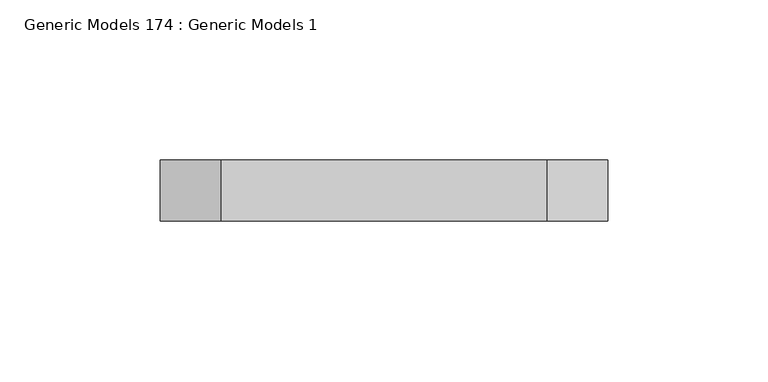
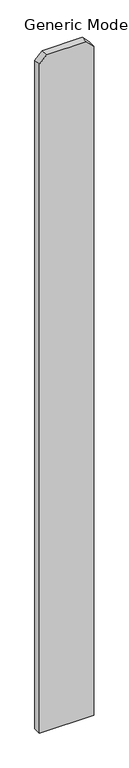
"""IFC4 building model written with IfcOpenShell, lengths in millimetres: proxy geometry, Generic Models 174 : Generic Models 1."""

import ifcopenshell
import ifcopenshell.guid

model = None  # the IFC model being written
_history = None  # IfcOwnerHistory: only IFC2X3 demands one
_inside = {}  # id of a spatial element -> (the spatial element, [elements in it])
_under = {}  # id of a project, library or spatial element -> (it, [spatial elements below it])
_declared = {}  # id of a project -> (the project, [libraries it declares])
_typed = {}  # id of a type object -> (the type object, [elements of that type])
_made_of = {}  # id of a material, layer set ... -> (it, [elements and type objects made of it])


def new_model(schema):
    """Start an empty IFC model of exactly this schema.

    Asked for "IFC4X3", IfcOpenShell would pick the latest addendum, in which some entities
    have other attributes; the version numbers below select the first issue.
    IFC2X3 requires an IfcOwnerHistory on every rooted entity: one is made here for all.
    """
    global model, _history
    if schema == "IFC4X3":
        model = ifcopenshell.file(schema_version=(4, 3, 0, 0))
    else:
        model = ifcopenshell.file(schema=schema)
    _inside.clear()
    _under.clear()
    _declared.clear()
    _typed.clear()
    _made_of.clear()
    _history = None
    if model.schema == "IFC2X3":
        org = make("IfcOrganization", Name="unknown")
        user = make(
            "IfcPersonAndOrganization",
            ThePerson=make("IfcPerson", FamilyName="unknown"),
            TheOrganization=org,
        )
        app = make(
            "IfcApplication",
            ApplicationDeveloper=org,
            Version="unknown",
            ApplicationFullName="unknown",
            ApplicationIdentifier="unknown",
        )
        _history = make(
            "IfcOwnerHistory",
            OwningUser=user,
            OwningApplication=app,
            ChangeAction="ADDED",
            CreationDate=0,
        )
    return model


def make(cls, **values):
    """One entity of the class cls with the attributes given. An attribute that is None is left unset."""
    return model.create_entity(
        cls, **{name: value for name, value in values.items() if value is not None}
    )


def rooted(cls, **values):
    """An entity with a GlobalId (a new one), such as an element, a storey or a relation."""
    return make(cls, GlobalId=ifcopenshell.guid.new(), OwnerHistory=_history, **values)


def si_unit(unit_type, name, prefix=None):
    """IfcSIUnit, for example si_unit("LENGTHUNIT", "METRE", prefix="MILLI")."""
    return make("IfcSIUnit", UnitType=unit_type, Prefix=prefix, Name=name)


def assignment(units):
    """IfcUnitAssignment: the units of a project."""
    return None if units is None else make("IfcUnitAssignment", Units=units)


def point(xyz):
    """IfcCartesianPoint."""
    return None if xyz is None else make("IfcCartesianPoint", Coordinates=xyz)


def direction(xyz):
    """IfcDirection."""
    return None if xyz is None else make("IfcDirection", DirectionRatios=xyz)


def frame(location, z_axis=None, x_axis=None):
    """IfcAxis2Placement3D, a coordinate frame: its origin and axes. An axis left out is left unset."""
    return make(
        "IfcAxis2Placement3D",
        Location=point(location),
        Axis=direction(z_axis),
        RefDirection=direction(x_axis),
    )


def origin():
    """The frame at (0, 0, 0) with its axes left unset."""
    return frame((0.0, 0.0, 0.0))


def place(relative_to, where):
    """IfcLocalPlacement: puts the frame where relative to a parent placement (None: the world)."""
    return make(
        "IfcLocalPlacement", PlacementRelTo=relative_to, RelativePlacement=where
    )


def context(
    kind, dimensions, precision=None, world=None, true_north=None, identifier=None
):
    """IfcGeometricRepresentationContext, for example the 3D "Model" context."""
    return make(
        "IfcGeometricRepresentationContext",
        ContextIdentifier=identifier,
        ContextType=kind,
        CoordinateSpaceDimension=dimensions,
        Precision=precision,
        WorldCoordinateSystem=world,
        TrueNorth=true_north,
    )


def project(units=None, contexts=None):
    """IfcProject with its units and contexts."""
    return rooted(
        "IfcProject",
        Name="project",
        RepresentationContexts=contexts,
        UnitsInContext=assignment(units),
    )


def spatial(cls, under=None, at=None, **own):
    """A site, building, storey or space (cls), placed at a placement, below another one or the project."""
    s = rooted(cls, ObjectPlacement=at, **own)
    if under is not None:
        _under.setdefault(under.id(), (under, []))[1].append(s)
    return s


def polyline(points):
    """IfcPolyline through the points."""
    return make("IfcPolyline", Points=[point(p) for p in points])


def outline(outer, holes=None, kind="AREA"):
    """IfcArbitraryClosedProfileDef: a profile drawn as a closed curve; with holes, ...WithVoids."""
    if holes is None:
        return make("IfcArbitraryClosedProfileDef", ProfileType=kind, OuterCurve=outer)
    return make(
        "IfcArbitraryProfileDefWithVoids",
        ProfileType=kind,
        OuterCurve=outer,
        InnerCurves=holes,
    )


def extrude(swept, where, along, depth):
    """IfcExtrudedAreaSolid: the profile swept, set in the frame where, extruded along a direction by depth."""
    return make(
        "IfcExtrudedAreaSolid",
        SweptArea=swept,
        Position=where,
        ExtrudedDirection=direction(along),
        Depth=depth,
    )


def shape(context_of_items, identifier, shape_type, items):
    """IfcShapeRepresentation: the items that make up one representation, for example the "Body"."""
    return make(
        "IfcShapeRepresentation",
        ContextOfItems=context_of_items,
        RepresentationIdentifier=identifier,
        RepresentationType=shape_type,
        Items=items,
    )


def source(mapping_origin, context_of_items, identifier, shape_type, items):
    """IfcRepresentationMap: a shape defined once, which mapped items show again and again."""
    return make(
        "IfcRepresentationMap",
        MappingOrigin=mapping_origin,
        MappedRepresentation=shape(context_of_items, identifier, shape_type, items),
    )


def transform(
    local_origin,
    x_axis=None,
    y_axis=None,
    z_axis=None,
    scale=None,
    scale2=None,
    scale3=None,
    uniform=True,
):
    """IfcCartesianTransformationOperator3D, or its non-uniform kind. x_axis, y_axis, z_axis: its Axis1, 2, 3."""
    if uniform:
        return make(
            "IfcCartesianTransformationOperator3D",
            Axis1=direction(x_axis),
            Axis2=direction(y_axis),
            LocalOrigin=point(local_origin),
            Scale=scale,
            Axis3=direction(z_axis),
        )
    return make(
        "IfcCartesianTransformationOperator3DnonUniform",
        Axis1=direction(x_axis),
        Axis2=direction(y_axis),
        LocalOrigin=point(local_origin),
        Scale=scale,
        Axis3=direction(z_axis),
        Scale2=scale2,
        Scale3=scale3,
    )


def mapped(mapping_source, mapping_target):
    """IfcMappedItem: shows the shape of a source again, moved by a transform."""
    return make(
        "IfcMappedItem", MappingSource=mapping_source, MappingTarget=mapping_target
    )


def made_of(thing, what):
    """Note that an element or type object is made of a material, layer set ...; save() writes the relation."""
    if what is not None:
        _made_of.setdefault(what.id(), (what, []))[1].append(thing)
    return thing


def element(
    cls,
    number,
    at=None,
    inside=None,
    cuts=None,
    type_object=None,
    material=None,
    context=None,
    identifier="Body",
    shape_type=None,
    held_by="IfcProductDefinitionShape",
    body=None,
    shapes=None,
    **own,
):
    """One element of the class cls, such as IfcWall. Its Tag is "e" and its number.

    at: its placement. inside: the storey or other place that contains it. cuts: it is an
    opening in that element (IfcRelVoidsElement). A single representation is given by context,
    identifier, shape_type and body (its items); several are given by shapes. held_by: the class
    of the entity that holds the representations. save() writes the other relations.
    """
    e = rooted(cls, Tag="e%d" % number, ObjectPlacement=at, **own)
    if body is not None:
        shapes = [shape(context, identifier, shape_type, body)]
    if shapes is not None:
        e.Representation = make(held_by, Representations=shapes)
    if inside is not None:
        _inside.setdefault(inside.id(), (inside, []))[1].append(e)
    if cuts is not None:
        rooted(
            "IfcRelVoidsElement", RelatingBuildingElement=cuts, RelatedOpeningElement=e
        )
    if type_object is not None:
        _typed.setdefault(type_object.id(), (type_object, []))[1].append(e)
    return made_of(e, material)


def aggregate(whole, parts):
    """IfcRelAggregates: a whole, such as a stair, and the parts it consists of."""
    return rooted("IfcRelAggregates", RelatingObject=whole, RelatedObjects=parts)


def save(model, path):
    """Write the relations noted so far, then the file.

    IfcRelAggregates (storeys below a building ...), IfcRelContainedInSpatialStructure (elements
    in a storey), IfcRelDefinesByType, IfcRelAssociatesMaterial and IfcRelDeclares: one each for
    every whole, place, type object, material and project.
    """
    for whole, parts in _under.values():
        aggregate(whole, parts)
    for where, things in _inside.values():
        rooted(
            "IfcRelContainedInSpatialStructure",
            RelatedElements=things,
            RelatingStructure=where,
        )
    for kind, things in _typed.values():
        rooted("IfcRelDefinesByType", RelatedObjects=things, RelatingType=kind)
    for what, things in _made_of.values():
        rooted("IfcRelAssociatesMaterial", RelatedObjects=things, RelatingMaterial=what)
    for by, libraries in _declared.values():
        rooted("IfcRelDeclares", RelatingContext=by, RelatedDefinitions=libraries)
    model.write(path)


def generic_models_174_generic_models_1_71a4a4c7(model_context):
    return source(origin(), model_context, "Body", "SweptSolid", [
        extrude(outline(polyline([(76.2, -248286.5875), (1885.95, -248286.5875), (1905.0, -248305.6375), (1905.0, -248407.2375), (1885.95, -248426.2875), (76.2, -248426.2875), (76.2, -248286.5875)])), frame((0.0, 547.6875, 0.0), z_axis=(0.0, 1.0, 0.0), x_axis=(0.0, 0.0, 1.0)), (0.0, 0.0, 1.0), 19.05),
    ])


if __name__ == "__main__":
    model = new_model("IFC4")
    model_context = context("Model", 3, world=origin())
    ifc_project = project(units=[si_unit("LENGTHUNIT", "METRE", prefix="MILLI")], contexts=[model_context])
    site = spatial("IfcSite", under=ifc_project)
    building = spatial("IfcBuilding", under=site)
    placement = place(None, origin())
    generic_models_174_generic_models_1_shape = generic_models_174_generic_models_1_71a4a4c7(model_context)
    element("IfcBuildingElementProxy", 1, Name="Generic Models 174 : Generic Models 1", ObjectType="Generic Models 174 : Generic Models 1", at=placement, inside=building, context=model_context, shape_type="MappedRepresentation", body=[
        mapped(generic_models_174_generic_models_1_shape, transform((0.0, 0.0, 0.0), x_axis=(1.0, 0.0, 0.0), y_axis=(0.0, 1.0, 0.0), z_axis=(0.0, 0.0, 1.0))),
    ])
    save(model, "model.ifc")

# Revit data of these elements
# Element 1 (IfcBuildingElementProxy, "Generic Models 174 : Generic Models 1")
#   Materials on its faces: "VERTICAL 1X6 CEDAR PLANKS W/ CLEAR WOOD SEALER"
# Materials
#   "VERTICAL 1X6 CEDAR PLANKS W/ CLEAR WOOD SEALER": class "Wood", colour RGB 234 198 147, transparency 0, Description = "Pinus Echinata", Cost = 0
